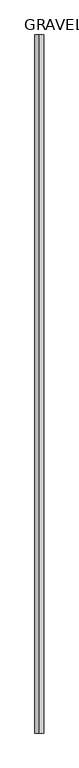
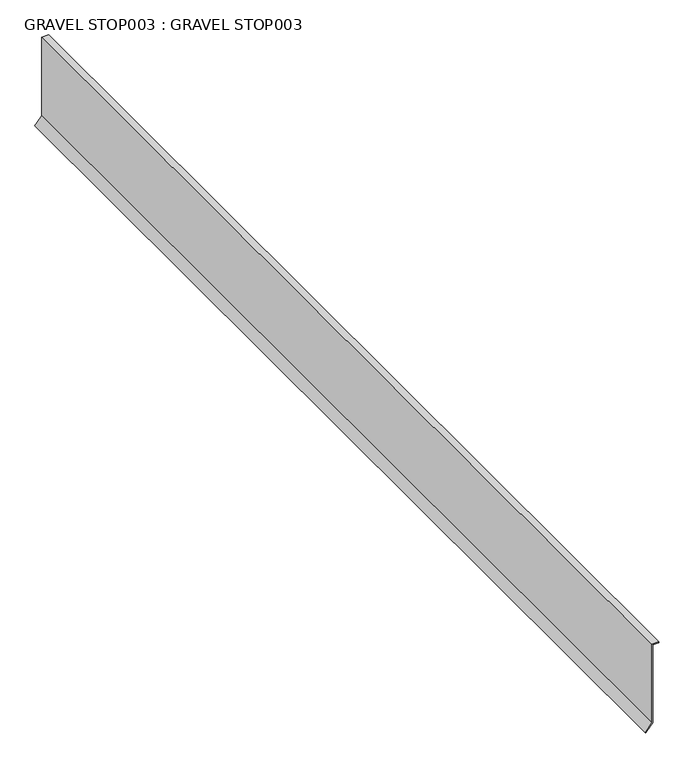
"""IFC4 building model written with IfcOpenShell, lengths in millimetres: proxy geometry, GRAVEL STOP003 : GRAVEL STOP003."""

from ifc_helpers import new_model, si_unit, frame, origin, place, context, project, spatial, polyline, outline, extrude, source, transform, mapped, element, save


def gravel_stop003_gravel_stop003_73d50619(model_context):
    return source(origin(), model_context, "Body", "SweptSolid", [
        extrude(outline(polyline([(40082.2407116, -5046.164524), (40081.3605882, -5045.0615204), (40097.4918556, -5032.189842), (40253.3245993, -5032.189842), (40253.3245993, -5020.4219233), (40254.7357103, -5020.4219233), (40254.7357103, -5033.600953), (40097.9858473, -5033.600953), (40082.2407116, -5046.164524)])), frame((0.0, -1052.8906573, 0.0), z_axis=(0.0, 1.0, 0.0), x_axis=(0.0, 0.0, 1.0)), (0.0, 0.0, 1.0), 2000.25),
    ])


if __name__ == "__main__":
    model = new_model("IFC4")
    model_context = context("Model", 3, world=origin())
    ifc_project = project(units=[si_unit("LENGTHUNIT", "METRE", prefix="MILLI")], contexts=[model_context])
    site = spatial("IfcSite", under=ifc_project)
    building = spatial("IfcBuilding", under=site)
    placement = place(None, origin())
    gravel_stop003_gravel_stop003_shape = gravel_stop003_gravel_stop003_73d50619(model_context)
    element("IfcBuildingElementProxy", 1, Name="GRAVEL STOP003 : GRAVEL STOP003", ObjectType="GRAVEL STOP003 : GRAVEL STOP003", at=placement, inside=building, context=model_context, shape_type="MappedRepresentation", body=[
        mapped(gravel_stop003_gravel_stop003_shape, transform((0.0, 0.0, 0.0), x_axis=(1.0, 0.0, 0.0), y_axis=(0.0, 1.0, 0.0), z_axis=(0.0, 0.0, 1.0))),
    ])
    save(model, "model.ifc")

# Revit data of these elements
# Type "GRAVEL STOP003 : GRAVEL STOP003"
#   NameOverride = "GRAVEL STOP003"
# Element 1 (IfcBuildingElementProxy, "GRAVEL STOP003 : GRAVEL STOP003")
#   Materials on its faces: "GRAVEL STOP REQUIRED WITH GRAVEL SURFACE SYSTEMS"
# Materials
#   "GRAVEL STOP REQUIRED WITH GRAVEL SURFACE SYSTEMS": class "Unassigned", colour RGB 170 170 127, transparency 0
